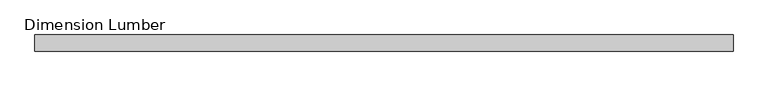
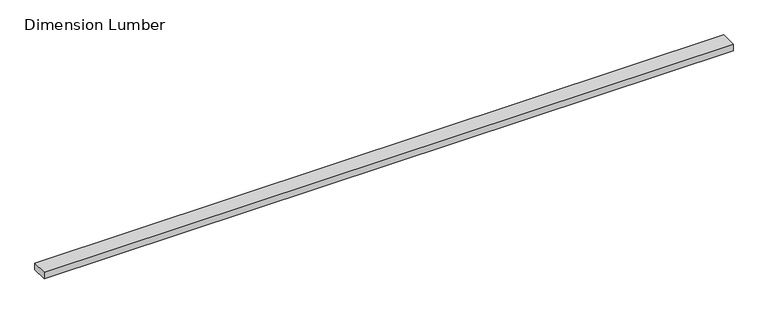
"""IFC4 building model written with IfcOpenShell, lengths in millimetres: beam geometry, Dimension Lumber : Top Supporting Lumbers."""

from ifc_helpers import new_model, si_unit, frame, origin, place, context, project, spatial, polyline, outline, extrude, source, transform, mapped, element, save


def dimension_lumber_39962a34(model_context):
    return source(origin(), model_context, "Body", "SweptSolid", [
        extrude(outline(polyline([(1941.5125, 44.45), (1941.5125, -44.45), (-1895.475, -44.45), (-1895.475, 44.45), (1941.5125, 44.45)])), frame((0.0, 0.0, -19.05), z_axis=(0.0, 0.0, 1.0), x_axis=(1.0, 0.0, 0.0)), (0.0, 0.0, 1.0), 38.1),
    ])


if __name__ == "__main__":
    model = new_model("IFC4")
    model_context = context("Model", 3, world=origin())
    ifc_project = project(units=[si_unit("LENGTHUNIT", "METRE", prefix="MILLI")], contexts=[model_context])
    site = spatial("IfcSite", under=ifc_project)
    building = spatial("IfcBuilding", under=site)
    placement = place(None, origin())
    dimension_lumber_shape = dimension_lumber_39962a34(model_context)
    element("IfcBeam", 1, ObjectType="Dimension Lumber : Top Supporting Lumbers", at=placement, inside=building, context=model_context, shape_type="MappedRepresentation", body=[
        mapped(dimension_lumber_shape, transform((0.0, 0.0, 0.0), x_axis=(1.0, 0.0, 0.0), y_axis=(0.0, 1.0, 0.0), z_axis=(0.0, 0.0, 1.0))),
    ])
    save(model, "model.ifc")

# Revit data of these elements
# Type "Dimension Lumber : Top Supporting Lumbers"
#   Assembly Code = "B10"
#   A = 0.0364583 SF
#   Length [instance default] = 5' - 0"
#   b = 0' - 3 1/2"
#   d = 0' - 1 1/2"
#   Structural Material [instance default] = Softwood, Lumber
# Element 1 (IfcBeam, "Dimension Lumber : Top Supporting Lumbers")
#   Structural Material = Douglas Fir #2
#   Materials on its faces: "Douglas Fir #2"
# Materials
#   "Softwood, Lumber": class "Wood", colour RGB 223 192 134, transparency 0, Description = "Pinus Echinata", Cost = 0
#   "Douglas Fir #2": class "Wood", colour RGB 223 192 134, transparency 0, Description = "Pinus Echinata", Cost = 0
